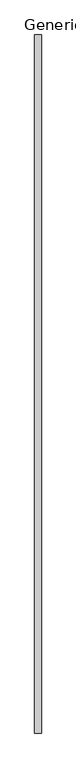
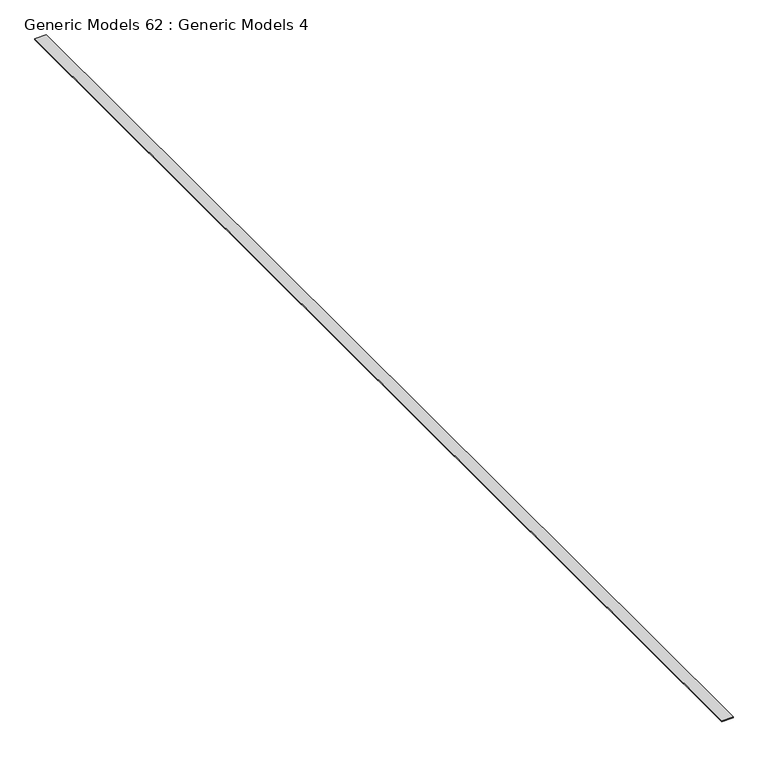
"""IFC4 building model written with IfcOpenShell, lengths in millimetres: proxy geometry, Generic Models 62 : Generic Models 4."""

from ifc_helpers import new_model, si_unit, frame, origin, place, context, project, spatial, polyline, outline, extrude, source, transform, mapped, element, save


def generic_models_62_generic_models_4_d58b3074(model_context):
    return source(origin(), model_context, "Body", "SweptSolid", [
        extrude(outline(polyline([(7347.0480051, -6864.9230338), (7169.2480051, -6864.9230338), (7169.2480051, 11778.6769662), (7347.0480051, 11778.6769662), (7347.0480051, -6864.9230338)])), frame((0.0, 0.0, 126524.8520404), z_axis=(0.0, 0.0, 1.0), x_axis=(1.0, 0.0, 0.0)), (0.0, 0.0, 1.0), 19.05),
    ])


if __name__ == "__main__":
    model = new_model("IFC4")
    model_context = context("Model", 3, world=origin())
    ifc_project = project(units=[si_unit("LENGTHUNIT", "METRE", prefix="MILLI")], contexts=[model_context])
    site = spatial("IfcSite", under=ifc_project)
    building = spatial("IfcBuilding", under=site)
    placement = place(None, origin())
    generic_models_62_generic_models_4_shape = generic_models_62_generic_models_4_d58b3074(model_context)
    element("IfcBuildingElementProxy", 1, Name="Generic Models 62 : Generic Models 4", ObjectType="Generic Models 62 : Generic Models 4", at=placement, inside=building, context=model_context, shape_type="MappedRepresentation", body=[
        mapped(generic_models_62_generic_models_4_shape, transform((0.0, 0.0, 0.0), x_axis=(1.0, 0.0, 0.0), y_axis=(0.0, 1.0, 0.0), z_axis=(0.0, 0.0, 1.0))),
    ])
    save(model, "model.ifc")

# Revit data of these elements
# Element 1 (IfcBuildingElementProxy, "Generic Models 62 : Generic Models 4")
#   Materials on its faces: "_CDX PLYWOOD - SEE STRUCT DWGs"
# Materials
#   "_CDX PLYWOOD - SEE STRUCT DWGs": class "Generic", colour RGB 98 75 74, transparency 0, Cost = 0
